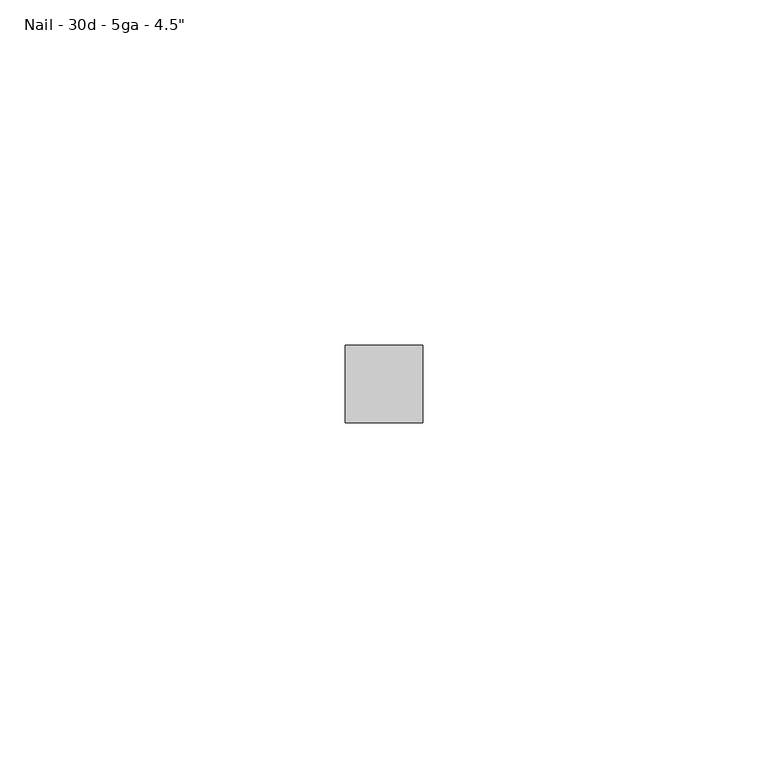
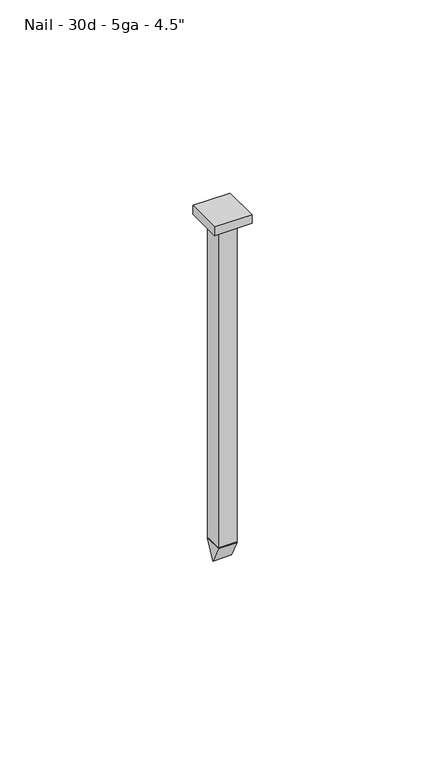
"""IFC4 building model written with IfcOpenShell, lengths in millimetres: fastener geometry."""

import ifcopenshell
import ifcopenshell.guid

model = None  # the IFC model being written
_history = None  # IfcOwnerHistory: only IFC2X3 demands one
_inside = {}  # id of a spatial element -> (the spatial element, [elements in it])
_under = {}  # id of a project, library or spatial element -> (it, [spatial elements below it])
_declared = {}  # id of a project -> (the project, [libraries it declares])
_typed = {}  # id of a type object -> (the type object, [elements of that type])
_made_of = {}  # id of a material, layer set ... -> (it, [elements and type objects made of it])


def new_model(schema):
    """Start an empty IFC model of exactly this schema.

    Asked for "IFC4X3", IfcOpenShell would pick the latest addendum, in which some entities
    have other attributes; the version numbers below select the first issue.
    IFC2X3 requires an IfcOwnerHistory on every rooted entity: one is made here for all.
    """
    global model, _history
    if schema == "IFC4X3":
        model = ifcopenshell.file(schema_version=(4, 3, 0, 0))
    else:
        model = ifcopenshell.file(schema=schema)
    _inside.clear()
    _under.clear()
    _declared.clear()
    _typed.clear()
    _made_of.clear()
    _history = None
    if model.schema == "IFC2X3":
        org = make("IfcOrganization", Name="unknown")
        user = make(
            "IfcPersonAndOrganization",
            ThePerson=make("IfcPerson", FamilyName="unknown"),
            TheOrganization=org,
        )
        app = make(
            "IfcApplication",
            ApplicationDeveloper=org,
            Version="unknown",
            ApplicationFullName="unknown",
            ApplicationIdentifier="unknown",
        )
        _history = make(
            "IfcOwnerHistory",
            OwningUser=user,
            OwningApplication=app,
            ChangeAction="ADDED",
            CreationDate=0,
        )
    return model


def make(cls, **values):
    """One entity of the class cls with the attributes given. An attribute that is None is left unset."""
    return model.create_entity(
        cls, **{name: value for name, value in values.items() if value is not None}
    )


def rooted(cls, **values):
    """An entity with a GlobalId (a new one), such as an element, a storey or a relation."""
    return make(cls, GlobalId=ifcopenshell.guid.new(), OwnerHistory=_history, **values)


def si_unit(unit_type, name, prefix=None):
    """IfcSIUnit, for example si_unit("LENGTHUNIT", "METRE", prefix="MILLI")."""
    return make("IfcSIUnit", UnitType=unit_type, Prefix=prefix, Name=name)


def assignment(units):
    """IfcUnitAssignment: the units of a project."""
    return None if units is None else make("IfcUnitAssignment", Units=units)


def point(xyz):
    """IfcCartesianPoint."""
    return None if xyz is None else make("IfcCartesianPoint", Coordinates=xyz)


def direction(xyz):
    """IfcDirection."""
    return None if xyz is None else make("IfcDirection", DirectionRatios=xyz)


def frame(location, z_axis=None, x_axis=None):
    """IfcAxis2Placement3D, a coordinate frame: its origin and axes. An axis left out is left unset."""
    return make(
        "IfcAxis2Placement3D",
        Location=point(location),
        Axis=direction(z_axis),
        RefDirection=direction(x_axis),
    )


def origin():
    """The frame at (0, 0, 0) with its axes left unset."""
    return frame((0.0, 0.0, 0.0))


def origin_with_axes():
    """The frame at (0, 0, 0) with the z axis (0, 0, 1) and the x axis (1, 0, 0) written out."""
    return frame((0.0, 0.0, 0.0), z_axis=(0.0, 0.0, 1.0), x_axis=(1.0, 0.0, 0.0))


def place(relative_to, where):
    """IfcLocalPlacement: puts the frame where relative to a parent placement (None: the world)."""
    return make(
        "IfcLocalPlacement", PlacementRelTo=relative_to, RelativePlacement=where
    )


def context(
    kind, dimensions, precision=None, world=None, true_north=None, identifier=None
):
    """IfcGeometricRepresentationContext, for example the 3D "Model" context."""
    return make(
        "IfcGeometricRepresentationContext",
        ContextIdentifier=identifier,
        ContextType=kind,
        CoordinateSpaceDimension=dimensions,
        Precision=precision,
        WorldCoordinateSystem=world,
        TrueNorth=true_north,
    )


def project(units=None, contexts=None):
    """IfcProject with its units and contexts."""
    return rooted(
        "IfcProject",
        Name="project",
        RepresentationContexts=contexts,
        UnitsInContext=assignment(units),
    )


def spatial(cls, under=None, at=None, **own):
    """A site, building, storey or space (cls), placed at a placement, below another one or the project."""
    s = rooted(cls, ObjectPlacement=at, **own)
    if under is not None:
        _under.setdefault(under.id(), (under, []))[1].append(s)
    return s


def polyline(points):
    """IfcPolyline through the points."""
    return make("IfcPolyline", Points=[point(p) for p in points])


def outline(outer, holes=None, kind="AREA"):
    """IfcArbitraryClosedProfileDef: a profile drawn as a closed curve; with holes, ...WithVoids."""
    if holes is None:
        return make("IfcArbitraryClosedProfileDef", ProfileType=kind, OuterCurve=outer)
    return make(
        "IfcArbitraryProfileDefWithVoids",
        ProfileType=kind,
        OuterCurve=outer,
        InnerCurves=holes,
    )


def extrude(swept, where, along, depth):
    """IfcExtrudedAreaSolid: the profile swept, set in the frame where, extruded along a direction by depth."""
    return make(
        "IfcExtrudedAreaSolid",
        SweptArea=swept,
        Position=where,
        ExtrudedDirection=direction(along),
        Depth=depth,
    )


def shape(context_of_items, identifier, shape_type, items):
    """IfcShapeRepresentation: the items that make up one representation, for example the "Body"."""
    return make(
        "IfcShapeRepresentation",
        ContextOfItems=context_of_items,
        RepresentationIdentifier=identifier,
        RepresentationType=shape_type,
        Items=items,
    )


def source(mapping_origin, context_of_items, identifier, shape_type, items):
    """IfcRepresentationMap: a shape defined once, which mapped items show again and again."""
    return make(
        "IfcRepresentationMap",
        MappingOrigin=mapping_origin,
        MappedRepresentation=shape(context_of_items, identifier, shape_type, items),
    )


def transform(
    local_origin,
    x_axis=None,
    y_axis=None,
    z_axis=None,
    scale=None,
    scale2=None,
    scale3=None,
    uniform=True,
):
    """IfcCartesianTransformationOperator3D, or its non-uniform kind. x_axis, y_axis, z_axis: its Axis1, 2, 3."""
    if uniform:
        return make(
            "IfcCartesianTransformationOperator3D",
            Axis1=direction(x_axis),
            Axis2=direction(y_axis),
            LocalOrigin=point(local_origin),
            Scale=scale,
            Axis3=direction(z_axis),
        )
    return make(
        "IfcCartesianTransformationOperator3DnonUniform",
        Axis1=direction(x_axis),
        Axis2=direction(y_axis),
        LocalOrigin=point(local_origin),
        Scale=scale,
        Axis3=direction(z_axis),
        Scale2=scale2,
        Scale3=scale3,
    )


def mapped(mapping_source, mapping_target):
    """IfcMappedItem: shows the shape of a source again, moved by a transform."""
    return make(
        "IfcMappedItem", MappingSource=mapping_source, MappingTarget=mapping_target
    )


def made_of(thing, what):
    """Note that an element or type object is made of a material, layer set ...; save() writes the relation."""
    if what is not None:
        _made_of.setdefault(what.id(), (what, []))[1].append(thing)
    return thing


def element(
    cls,
    number,
    at=None,
    inside=None,
    cuts=None,
    type_object=None,
    material=None,
    context=None,
    identifier="Body",
    shape_type=None,
    held_by="IfcProductDefinitionShape",
    body=None,
    shapes=None,
    **own,
):
    """One element of the class cls, such as IfcWall. Its Tag is "e" and its number.

    at: its placement. inside: the storey or other place that contains it. cuts: it is an
    opening in that element (IfcRelVoidsElement). A single representation is given by context,
    identifier, shape_type and body (its items); several are given by shapes. held_by: the class
    of the entity that holds the representations. save() writes the other relations.
    """
    e = rooted(cls, Tag="e%d" % number, ObjectPlacement=at, **own)
    if body is not None:
        shapes = [shape(context, identifier, shape_type, body)]
    if shapes is not None:
        e.Representation = make(held_by, Representations=shapes)
    if inside is not None:
        _inside.setdefault(inside.id(), (inside, []))[1].append(e)
    if cuts is not None:
        rooted(
            "IfcRelVoidsElement", RelatingBuildingElement=cuts, RelatedOpeningElement=e
        )
    if type_object is not None:
        _typed.setdefault(type_object.id(), (type_object, []))[1].append(e)
    return made_of(e, material)


def aggregate(whole, parts):
    """IfcRelAggregates: a whole, such as a stair, and the parts it consists of."""
    return rooted("IfcRelAggregates", RelatingObject=whole, RelatedObjects=parts)


def save(model, path):
    """Write the relations noted so far, then the file.

    IfcRelAggregates (storeys below a building ...), IfcRelContainedInSpatialStructure (elements
    in a storey), IfcRelDefinesByType, IfcRelAssociatesMaterial and IfcRelDeclares: one each for
    every whole, place, type object, material and project.
    """
    for whole, parts in _under.values():
        aggregate(whole, parts)
    for where, things in _inside.values():
        rooted(
            "IfcRelContainedInSpatialStructure",
            RelatedElements=things,
            RelatingStructure=where,
        )
    for kind, things in _typed.values():
        rooted("IfcRelDefinesByType", RelatedObjects=things, RelatingType=kind)
    for what, things in _made_of.values():
        rooted("IfcRelAssociatesMaterial", RelatedObjects=things, RelatingMaterial=what)
    for by, libraries in _declared.values():
        rooted("IfcRelDeclares", RelatingContext=by, RelatedDefinitions=libraries)
    model.write(path)


def fastener_3e67c611(model_context):
    return source(origin(), model_context, "Body", "SweptSolid", [
        extrude(outline(polyline([(0.0, -107.188), (-2.794, -101.6), (2.794, -101.6), (0.0, -107.188)])), frame((-2.794, 0.0, 0.0), z_axis=(1.0, 0.0, 0.0), x_axis=(0.0, 1.0, 0.0)), (0.0, 0.0, 1.0), 5.588),
        extrude(outline(polyline([(-5.588, -5.588), (-5.588, 5.588), (5.588, 5.588), (5.588, -5.588), (-5.588, -5.588)])), origin_with_axes(), (0.0, 0.0, 1.0), 2.794),
        extrude(outline(polyline([(-2.794, 2.794), (2.794, 2.794), (2.794, -2.794), (-2.794, -2.794), (-2.794, 2.794)])), frame((0.0, 0.0, -101.6), z_axis=(0.0, 0.0, 1.0), x_axis=(1.0, 0.0, 0.0)), (0.0, 0.0, 1.0), 101.6),
    ])


if __name__ == "__main__":
    model = new_model("IFC4")
    model_context = context("Model", 3, world=origin())
    ifc_project = project(units=[si_unit("LENGTHUNIT", "METRE", prefix="MILLI")], contexts=[model_context])
    site = spatial("IfcSite", under=ifc_project)
    building = spatial("IfcBuilding", under=site)
    placement = place(None, origin())
    fastener_shape = fastener_3e67c611(model_context)
    element("IfcFastener", 1, ObjectType="060523 - W_P_C - Fastenings - Generic - SQUARE : Nail - 30d - 5ga - 4.5\"", at=placement, inside=building, context=model_context, shape_type="MappedRepresentation", body=[
        mapped(fastener_shape, transform((0.0, 0.0, 0.0), x_axis=(1.0, 0.0, 0.0), y_axis=(0.0, 1.0, 0.0), z_axis=(0.0, 0.0, 1.0))),
    ])
    save(model, "model.ifc")

# Revit data of these elements
# Type "060523 - W_P_C - Fastenings - Generic - SQUARE : Nail - 30d - 5ga - 4.5\""
#   Washer_Thickness = 0' - 0.00333"
#   Washer Radius = 0' - 0.12"
#   Washer Offset - Head = 0' - 0"
#   Washer Offset = 0' - 0"
#   Thickness_of_Substrate [instance default] = 0' - 1"
#   Side = 0' - 0 37/64"
#   Radius = 0' - 0.11"
#   Length [instance default] = 0' - 4 1/2"
#   Head Size = 0' - 1"
#   Head Radius = 0' - 0 1/2"
#   Head Height = 0' - 0.01"
#   Double Diameter = 0' - 0.44"
#   Diameter = 0' - 0.22"
#   Default Elevation = 4' - 0"
#   Washer_Nut_Visibility = no
#   Washer_Head_Visibility = no
#   Round_Head_Visibility = yes
#   Point Visibility = yes
#   Nut_Visibility = no
#   Hex_Head_Visiblilty = no
#   Washer Material = none
#   Bolt Material (Size) = AT SILL - FASTENER AT 24" O.C.
# Element 1 (IfcFastener, "060523 - W_P_C - Fastenings - Generic - SQUARE : Nail - 30d - 5ga - 4.5\"")
#   Length = 0' - 4"
# Materials
#   "AT SILL - FASTENER AT 24\" O.C.": class "Generic", colour RGB 120 120 120, transparency 0, Cost = 0
